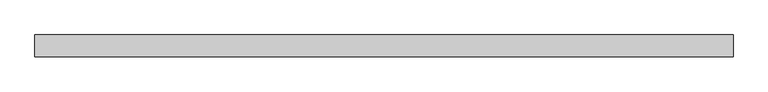
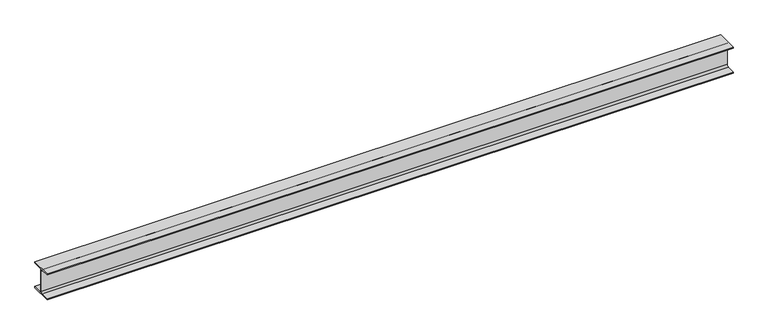
"""IFC4 building model written with IfcOpenShell, lengths in millimetres: beam geometry, 0912_Steel Framing_H-KSD3502 : H_SB_AR_S02_H-194x150x6x9_Platform."""

from ifc_helpers import new_model, si_unit, point, frame, frame_2d, origin, place, context, project, spatial, polyline, circle_curve, trimmed, segment, composite_curve, outline, extrude, source, transform, mapped, element, save


def beam_719db1ac(model_context):
    return source(origin(), model_context, "Body", "SweptSolid", [
        extrude(outline(composite_curve([segment(polyline([(75.0, -88.0), (75.0, -97.0), (-75.0, -97.0), (-75.0, -88.0), (-16.0, -88.0)]), True, "CONTINUOUS"), segment(trimmed(circle_curve(frame_2d((-16.0, -75.0)), 13.0), [point((-16.0, -88.0))], [point((-3.0, -75.0))], True, "CARTESIAN"), True, "CONTINUOUS"), segment(polyline([(-3.0, -75.0), (-3.0, 75.0)]), True, "CONTINUOUS"), segment(trimmed(circle_curve(frame_2d((-16.0, 75.0)), 13.0), [point((-3.0, 75.0))], [point((-16.0, 88.0))], True, "CARTESIAN"), True, "CONTINUOUS"), segment(polyline([(-16.0, 88.0), (-75.0, 88.0), (-75.0, 97.0), (75.0, 97.0), (75.0, 88.0), (16.0, 88.0)]), True, "CONTINUOUS"), segment(trimmed(circle_curve(frame_2d((16.0, 75.0)), 13.0), [point((16.0, 88.0))], [point((3.0, 75.0))], True, "CARTESIAN"), True, "CONTINUOUS"), segment(polyline([(3.0, 75.0), (3.0, -75.0)]), True, "CONTINUOUS"), segment(trimmed(circle_curve(frame_2d((16.0, -75.0)), 13.0), [point((3.0, -75.0))], [point((16.0, -88.0))], True, "CARTESIAN"), True, "CONTINUOUS"), segment(polyline([(16.0, -88.0), (75.0, -88.0)]), True, "CONTINUOUS")], self_intersect=False)), frame((-2412.3, 0.0, 0.0), z_axis=(1.0, 0.0, 0.0), x_axis=(0.0, 1.0, 0.0)), (0.0, 0.0, 1.0), 4824.6),
    ])


if __name__ == "__main__":
    model = new_model("IFC4")
    model_context = context("Model", 3, world=origin())
    ifc_project = project(units=[si_unit("LENGTHUNIT", "METRE", prefix="MILLI")], contexts=[model_context])
    site = spatial("IfcSite", under=ifc_project)
    building = spatial("IfcBuilding", under=site)
    placement = place(None, origin())
    beam_shape = beam_719db1ac(model_context)
    element("IfcBeam", 1, ObjectType="0912_Steel Framing_H-KSD3502 : H_SB_AR_S02_H-194x150x6x9_Platform", at=placement, inside=building, context=model_context, shape_type="MappedRepresentation", body=[
        mapped(beam_shape, transform((0.0, 0.0, 0.0), x_axis=(1.0, 0.0, 0.0), y_axis=(0.0, 1.0, 0.0), z_axis=(0.0, 0.0, 1.0))),
    ])
    save(model, "model.ifc")

# Revit data of these elements
# Type "0912_Steel Framing_H-KSD3502 : H_SB_AR_S02_H-194x150x6x9_Platform"
#   H_Q'ty Cal Type Tag = "SB-Q2"
#   H_WM Code_1 = "S01AA073-00001 |  | TON | Main Steel Structure Fabrication Work | Shelter/Building | Medium Steel - Standard |  |  |  |  |  |  | Material: (   ) | (90)KG/M>Weight≥(30)KG/M | S01AA073-00001 Main Steel Structure Fabrication Work Shelter/Building Medium Steel - Standard         | - Material: ( ASTM A36 )\n- (90)KG/M>Weight≥(30)KG/M"
#   H_WM Code_2 = "S03AA083-00001 |  | TON | Main Steel Structure Erection Work | Shelter/Building | Medium Steel |  |  |  |  |  |  | Material: (   ) | S03AA083-00001 Main Steel Structure Erection Work Shelter/Building Medium Steel         | - Material: ( ASTM A36 )"
#   H_WM Code_3 = "S01AA009-00001 |  | TON | Main Steel Structure Fabrication Work | Shelter/Building | Plates - Gusset, Stiffener, ETC | Material: (   ) | S01AA009-00001 Main Steel Structure Fabrication Work Shelter/Building Plates - Gusset, Stiffener, ETC         |"
#   H_WM Code_4 = "S41AA051-00001 |  | M2 | Steel Structure Paint Work | Shelter/Building | for Non-Fireproofed Steel Surface |  |  |  |  |  |  | Material: (   ) | S41AA051-00001 Steel Structure Paint Work Shelter/Building for Non-Fireproofed Steel Surface         |"
#   Width = 15.0 cm
#   Web Thickness = 0.6 cm
#   Web Fillet = 1.3 cm
#   Warping Constant = 43316.0 cm⁶
#   W = 0
#   Torsional Moment of Inertia = 8.622 cm⁴
#   Section Area = 39.01 cm²
#   Plastic Modulus weak axis = 104.0 cm³
#   Plastic Modulus strong axis = 309.0 cm³
#   Perimeter = 0.95 m²/m
#   Nominal Weight = 30.60 kgf/m
#   Moment of Inertia weak axis = 507.00 cm⁴
#   Moment of Inertia strong axis = 2690.00 cm⁴
#   Height = 19.4 cm
#   Flange Thickness = 0.9 cm
#   Elastic Modulus weak axis = 67.6 cm³
#   Elastic Modulus strong axis = 277.0 cm³
#   Centroid Vertical = 9.7 cm
#   Centroid Horizontal = 7.5 cm
#   Ix = 26900000
#   Length [instance default] = 1524 mm
#   Zx = 309000
#   b = 150 mm
#   h = 194 mm
#   r = 13 mm
#   s = 6 mm
#   t = 9 mm
#   A = 0.003901 m²
#   Structural Material [instance default] = Steel, 45-345
#   Assembly Code = ""
# Element 1 (IfcBeam, "0912_Steel Framing_H-KSD3502 : H_SB_AR_S02_H-194x150x6x9_Platform")
#   Materials on its faces: "Steel, 45-345"
# Materials
#   "Steel, 45-345": class "Metal", colour RGB 189 187 185, transparency 0, Description = "Steel 345 MPa", Cost = 0
